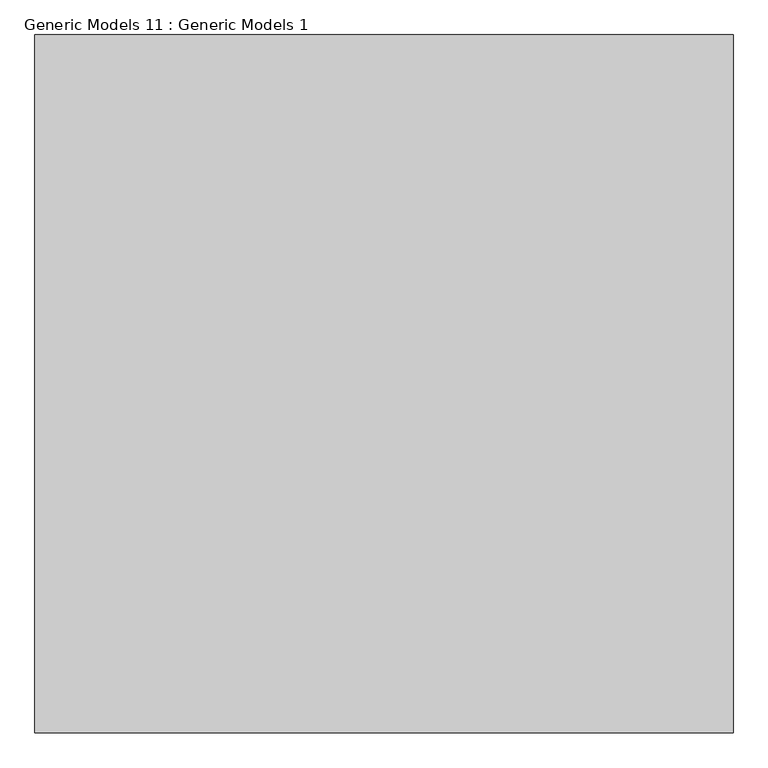
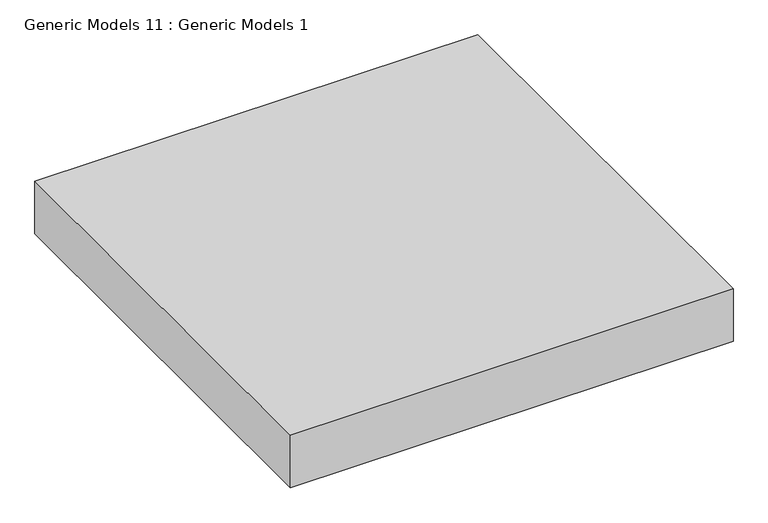
"""IFC4 building model written with IfcOpenShell, lengths in millimetres: proxy geometry, Generic Models 11 : Generic Models 1."""

import ifcopenshell
import ifcopenshell.guid

model = None  # the IFC model being written
_history = None  # IfcOwnerHistory: only IFC2X3 demands one
_inside = {}  # id of a spatial element -> (the spatial element, [elements in it])
_under = {}  # id of a project, library or spatial element -> (it, [spatial elements below it])
_declared = {}  # id of a project -> (the project, [libraries it declares])
_typed = {}  # id of a type object -> (the type object, [elements of that type])
_made_of = {}  # id of a material, layer set ... -> (it, [elements and type objects made of it])


def new_model(schema):
    """Start an empty IFC model of exactly this schema.

    Asked for "IFC4X3", IfcOpenShell would pick the latest addendum, in which some entities
    have other attributes; the version numbers below select the first issue.
    IFC2X3 requires an IfcOwnerHistory on every rooted entity: one is made here for all.
    """
    global model, _history
    if schema == "IFC4X3":
        model = ifcopenshell.file(schema_version=(4, 3, 0, 0))
    else:
        model = ifcopenshell.file(schema=schema)
    _inside.clear()
    _under.clear()
    _declared.clear()
    _typed.clear()
    _made_of.clear()
    _history = None
    if model.schema == "IFC2X3":
        org = make("IfcOrganization", Name="unknown")
        user = make(
            "IfcPersonAndOrganization",
            ThePerson=make("IfcPerson", FamilyName="unknown"),
            TheOrganization=org,
        )
        app = make(
            "IfcApplication",
            ApplicationDeveloper=org,
            Version="unknown",
            ApplicationFullName="unknown",
            ApplicationIdentifier="unknown",
        )
        _history = make(
            "IfcOwnerHistory",
            OwningUser=user,
            OwningApplication=app,
            ChangeAction="ADDED",
            CreationDate=0,
        )
    return model


def make(cls, **values):
    """One entity of the class cls with the attributes given. An attribute that is None is left unset."""
    return model.create_entity(
        cls, **{name: value for name, value in values.items() if value is not None}
    )


def rooted(cls, **values):
    """An entity with a GlobalId (a new one), such as an element, a storey or a relation."""
    return make(cls, GlobalId=ifcopenshell.guid.new(), OwnerHistory=_history, **values)


def si_unit(unit_type, name, prefix=None):
    """IfcSIUnit, for example si_unit("LENGTHUNIT", "METRE", prefix="MILLI")."""
    return make("IfcSIUnit", UnitType=unit_type, Prefix=prefix, Name=name)


def assignment(units):
    """IfcUnitAssignment: the units of a project."""
    return None if units is None else make("IfcUnitAssignment", Units=units)


def point(xyz):
    """IfcCartesianPoint."""
    return None if xyz is None else make("IfcCartesianPoint", Coordinates=xyz)


def direction(xyz):
    """IfcDirection."""
    return None if xyz is None else make("IfcDirection", DirectionRatios=xyz)


def frame(location, z_axis=None, x_axis=None):
    """IfcAxis2Placement3D, a coordinate frame: its origin and axes. An axis left out is left unset."""
    return make(
        "IfcAxis2Placement3D",
        Location=point(location),
        Axis=direction(z_axis),
        RefDirection=direction(x_axis),
    )


def origin():
    """The frame at (0, 0, 0) with its axes left unset."""
    return frame((0.0, 0.0, 0.0))


def place(relative_to, where):
    """IfcLocalPlacement: puts the frame where relative to a parent placement (None: the world)."""
    return make(
        "IfcLocalPlacement", PlacementRelTo=relative_to, RelativePlacement=where
    )


def context(
    kind, dimensions, precision=None, world=None, true_north=None, identifier=None
):
    """IfcGeometricRepresentationContext, for example the 3D "Model" context."""
    return make(
        "IfcGeometricRepresentationContext",
        ContextIdentifier=identifier,
        ContextType=kind,
        CoordinateSpaceDimension=dimensions,
        Precision=precision,
        WorldCoordinateSystem=world,
        TrueNorth=true_north,
    )


def project(units=None, contexts=None):
    """IfcProject with its units and contexts."""
    return rooted(
        "IfcProject",
        Name="project",
        RepresentationContexts=contexts,
        UnitsInContext=assignment(units),
    )


def spatial(cls, under=None, at=None, **own):
    """A site, building, storey or space (cls), placed at a placement, below another one or the project."""
    s = rooted(cls, ObjectPlacement=at, **own)
    if under is not None:
        _under.setdefault(under.id(), (under, []))[1].append(s)
    return s


def polyline(points):
    """IfcPolyline through the points."""
    return make("IfcPolyline", Points=[point(p) for p in points])


def outline(outer, holes=None, kind="AREA"):
    """IfcArbitraryClosedProfileDef: a profile drawn as a closed curve; with holes, ...WithVoids."""
    if holes is None:
        return make("IfcArbitraryClosedProfileDef", ProfileType=kind, OuterCurve=outer)
    return make(
        "IfcArbitraryProfileDefWithVoids",
        ProfileType=kind,
        OuterCurve=outer,
        InnerCurves=holes,
    )


def extrude(swept, where, along, depth):
    """IfcExtrudedAreaSolid: the profile swept, set in the frame where, extruded along a direction by depth."""
    return make(
        "IfcExtrudedAreaSolid",
        SweptArea=swept,
        Position=where,
        ExtrudedDirection=direction(along),
        Depth=depth,
    )


def shape(context_of_items, identifier, shape_type, items):
    """IfcShapeRepresentation: the items that make up one representation, for example the "Body"."""
    return make(
        "IfcShapeRepresentation",
        ContextOfItems=context_of_items,
        RepresentationIdentifier=identifier,
        RepresentationType=shape_type,
        Items=items,
    )


def source(mapping_origin, context_of_items, identifier, shape_type, items):
    """IfcRepresentationMap: a shape defined once, which mapped items show again and again."""
    return make(
        "IfcRepresentationMap",
        MappingOrigin=mapping_origin,
        MappedRepresentation=shape(context_of_items, identifier, shape_type, items),
    )


def transform(
    local_origin,
    x_axis=None,
    y_axis=None,
    z_axis=None,
    scale=None,
    scale2=None,
    scale3=None,
    uniform=True,
):
    """IfcCartesianTransformationOperator3D, or its non-uniform kind. x_axis, y_axis, z_axis: its Axis1, 2, 3."""
    if uniform:
        return make(
            "IfcCartesianTransformationOperator3D",
            Axis1=direction(x_axis),
            Axis2=direction(y_axis),
            LocalOrigin=point(local_origin),
            Scale=scale,
            Axis3=direction(z_axis),
        )
    return make(
        "IfcCartesianTransformationOperator3DnonUniform",
        Axis1=direction(x_axis),
        Axis2=direction(y_axis),
        LocalOrigin=point(local_origin),
        Scale=scale,
        Axis3=direction(z_axis),
        Scale2=scale2,
        Scale3=scale3,
    )


def mapped(mapping_source, mapping_target):
    """IfcMappedItem: shows the shape of a source again, moved by a transform."""
    return make(
        "IfcMappedItem", MappingSource=mapping_source, MappingTarget=mapping_target
    )


def made_of(thing, what):
    """Note that an element or type object is made of a material, layer set ...; save() writes the relation."""
    if what is not None:
        _made_of.setdefault(what.id(), (what, []))[1].append(thing)
    return thing


def element(
    cls,
    number,
    at=None,
    inside=None,
    cuts=None,
    type_object=None,
    material=None,
    context=None,
    identifier="Body",
    shape_type=None,
    held_by="IfcProductDefinitionShape",
    body=None,
    shapes=None,
    **own,
):
    """One element of the class cls, such as IfcWall. Its Tag is "e" and its number.

    at: its placement. inside: the storey or other place that contains it. cuts: it is an
    opening in that element (IfcRelVoidsElement). A single representation is given by context,
    identifier, shape_type and body (its items); several are given by shapes. held_by: the class
    of the entity that holds the representations. save() writes the other relations.
    """
    e = rooted(cls, Tag="e%d" % number, ObjectPlacement=at, **own)
    if body is not None:
        shapes = [shape(context, identifier, shape_type, body)]
    if shapes is not None:
        e.Representation = make(held_by, Representations=shapes)
    if inside is not None:
        _inside.setdefault(inside.id(), (inside, []))[1].append(e)
    if cuts is not None:
        rooted(
            "IfcRelVoidsElement", RelatingBuildingElement=cuts, RelatedOpeningElement=e
        )
    if type_object is not None:
        _typed.setdefault(type_object.id(), (type_object, []))[1].append(e)
    return made_of(e, material)


def aggregate(whole, parts):
    """IfcRelAggregates: a whole, such as a stair, and the parts it consists of."""
    return rooted("IfcRelAggregates", RelatingObject=whole, RelatedObjects=parts)


def save(model, path):
    """Write the relations noted so far, then the file.

    IfcRelAggregates (storeys below a building ...), IfcRelContainedInSpatialStructure (elements
    in a storey), IfcRelDefinesByType, IfcRelAssociatesMaterial and IfcRelDeclares: one each for
    every whole, place, type object, material and project.
    """
    for whole, parts in _under.values():
        aggregate(whole, parts)
    for where, things in _inside.values():
        rooted(
            "IfcRelContainedInSpatialStructure",
            RelatedElements=things,
            RelatingStructure=where,
        )
    for kind, things in _typed.values():
        rooted("IfcRelDefinesByType", RelatedObjects=things, RelatingType=kind)
    for what, things in _made_of.values():
        rooted("IfcRelAssociatesMaterial", RelatedObjects=things, RelatingMaterial=what)
    for by, libraries in _declared.values():
        rooted("IfcRelDeclares", RelatingContext=by, RelatedDefinitions=libraries)
    model.write(path)


def generic_models_11_generic_models_1_850b304e(model_context):
    return source(origin(), model_context, "Body", "SweptSolid", [
        extrude(outline(polyline([(50347.5625, 0.0), (49128.3625, 0.0), (49128.3625, 1219.2), (50347.5625, 1219.2), (50347.5625, 0.0)])), frame((0.0, 0.0, -152.4), z_axis=(0.0, 0.0, 1.0), x_axis=(1.0, 0.0, 0.0)), (0.0, 0.0, 1.0), 152.4),
    ])


if __name__ == "__main__":
    model = new_model("IFC4")
    model_context = context("Model", 3, world=origin())
    ifc_project = project(units=[si_unit("LENGTHUNIT", "METRE", prefix="MILLI")], contexts=[model_context])
    site = spatial("IfcSite", under=ifc_project)
    building = spatial("IfcBuilding", under=site)
    placement = place(None, origin())
    generic_models_11_generic_models_1_shape = generic_models_11_generic_models_1_850b304e(model_context)
    element("IfcBuildingElementProxy", 1, Name="Generic Models 11 : Generic Models 1", ObjectType="Generic Models 11 : Generic Models 1", at=placement, inside=building, context=model_context, shape_type="MappedRepresentation", body=[
        mapped(generic_models_11_generic_models_1_shape, transform((0.0, 0.0, 0.0), x_axis=(1.0, 0.0, 0.0), y_axis=(0.0, 1.0, 0.0), z_axis=(0.0, 0.0, 1.0))),
    ])
    save(model, "model.ifc")

# Revit data of these elements
# Element 1 (IfcBuildingElementProxy, "Generic Models 11 : Generic Models 1")
#   Materials on its faces: "STRUCTURAL FLOOR"
# Materials
#   "STRUCTURAL FLOOR": class "Concrete", colour RGB 129 132 118, transparency 0, Description = "Lightweight concrete", Cost = 0
